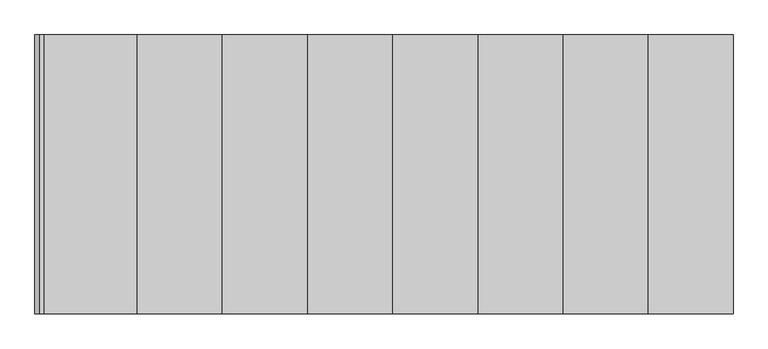
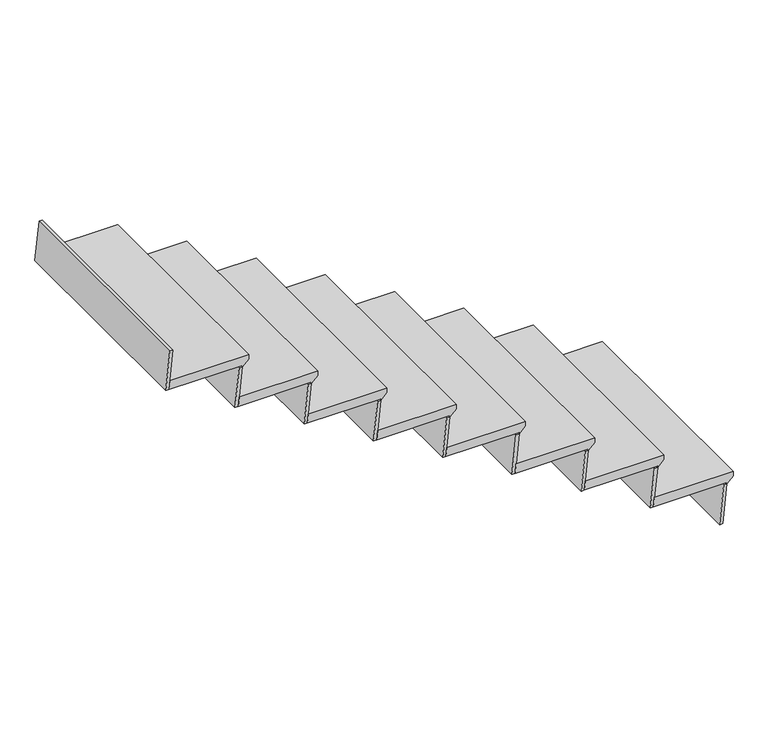
"""IFC4 building model written with IfcOpenShell, lengths in millimetres: stair flight geometry."""

import ifcopenshell
import ifcopenshell.guid

model = None  # the IFC model being written
_history = None  # IfcOwnerHistory: only IFC2X3 demands one
_inside = {}  # id of a spatial element -> (the spatial element, [elements in it])
_under = {}  # id of a project, library or spatial element -> (it, [spatial elements below it])
_declared = {}  # id of a project -> (the project, [libraries it declares])
_typed = {}  # id of a type object -> (the type object, [elements of that type])
_made_of = {}  # id of a material, layer set ... -> (it, [elements and type objects made of it])


def new_model(schema):
    """Start an empty IFC model of exactly this schema.

    Asked for "IFC4X3", IfcOpenShell would pick the latest addendum, in which some entities
    have other attributes; the version numbers below select the first issue.
    IFC2X3 requires an IfcOwnerHistory on every rooted entity: one is made here for all.
    """
    global model, _history
    if schema == "IFC4X3":
        model = ifcopenshell.file(schema_version=(4, 3, 0, 0))
    else:
        model = ifcopenshell.file(schema=schema)
    _inside.clear()
    _under.clear()
    _declared.clear()
    _typed.clear()
    _made_of.clear()
    _history = None
    if model.schema == "IFC2X3":
        org = make("IfcOrganization", Name="unknown")
        user = make(
            "IfcPersonAndOrganization",
            ThePerson=make("IfcPerson", FamilyName="unknown"),
            TheOrganization=org,
        )
        app = make(
            "IfcApplication",
            ApplicationDeveloper=org,
            Version="unknown",
            ApplicationFullName="unknown",
            ApplicationIdentifier="unknown",
        )
        _history = make(
            "IfcOwnerHistory",
            OwningUser=user,
            OwningApplication=app,
            ChangeAction="ADDED",
            CreationDate=0,
        )
    return model


def make(cls, **values):
    """One entity of the class cls with the attributes given. An attribute that is None is left unset."""
    return model.create_entity(
        cls, **{name: value for name, value in values.items() if value is not None}
    )


def rooted(cls, **values):
    """An entity with a GlobalId (a new one), such as an element, a storey or a relation."""
    return make(cls, GlobalId=ifcopenshell.guid.new(), OwnerHistory=_history, **values)


def si_unit(unit_type, name, prefix=None):
    """IfcSIUnit, for example si_unit("LENGTHUNIT", "METRE", prefix="MILLI")."""
    return make("IfcSIUnit", UnitType=unit_type, Prefix=prefix, Name=name)


def assignment(units):
    """IfcUnitAssignment: the units of a project."""
    return None if units is None else make("IfcUnitAssignment", Units=units)


def point(xyz):
    """IfcCartesianPoint."""
    return None if xyz is None else make("IfcCartesianPoint", Coordinates=xyz)


def direction(xyz):
    """IfcDirection."""
    return None if xyz is None else make("IfcDirection", DirectionRatios=xyz)


def frame(location, z_axis=None, x_axis=None):
    """IfcAxis2Placement3D, a coordinate frame: its origin and axes. An axis left out is left unset."""
    return make(
        "IfcAxis2Placement3D",
        Location=point(location),
        Axis=direction(z_axis),
        RefDirection=direction(x_axis),
    )


def origin():
    """The frame at (0, 0, 0) with its axes left unset."""
    return frame((0.0, 0.0, 0.0))


def place(relative_to, where):
    """IfcLocalPlacement: puts the frame where relative to a parent placement (None: the world)."""
    return make(
        "IfcLocalPlacement", PlacementRelTo=relative_to, RelativePlacement=where
    )


def context(
    kind, dimensions, precision=None, world=None, true_north=None, identifier=None
):
    """IfcGeometricRepresentationContext, for example the 3D "Model" context."""
    return make(
        "IfcGeometricRepresentationContext",
        ContextIdentifier=identifier,
        ContextType=kind,
        CoordinateSpaceDimension=dimensions,
        Precision=precision,
        WorldCoordinateSystem=world,
        TrueNorth=true_north,
    )


def project(units=None, contexts=None):
    """IfcProject with its units and contexts."""
    return rooted(
        "IfcProject",
        Name="project",
        RepresentationContexts=contexts,
        UnitsInContext=assignment(units),
    )


def spatial(cls, under=None, at=None, **own):
    """A site, building, storey or space (cls), placed at a placement, below another one or the project."""
    s = rooted(cls, ObjectPlacement=at, **own)
    if under is not None:
        _under.setdefault(under.id(), (under, []))[1].append(s)
    return s


def polyline(points):
    """IfcPolyline through the points."""
    return make("IfcPolyline", Points=[point(p) for p in points])


def outline(outer, holes=None, kind="AREA"):
    """IfcArbitraryClosedProfileDef: a profile drawn as a closed curve; with holes, ...WithVoids."""
    if holes is None:
        return make("IfcArbitraryClosedProfileDef", ProfileType=kind, OuterCurve=outer)
    return make(
        "IfcArbitraryProfileDefWithVoids",
        ProfileType=kind,
        OuterCurve=outer,
        InnerCurves=holes,
    )


def extrude(swept, where, along, depth):
    """IfcExtrudedAreaSolid: the profile swept, set in the frame where, extruded along a direction by depth."""
    return make(
        "IfcExtrudedAreaSolid",
        SweptArea=swept,
        Position=where,
        ExtrudedDirection=direction(along),
        Depth=depth,
    )


def shape(context_of_items, identifier, shape_type, items):
    """IfcShapeRepresentation: the items that make up one representation, for example the "Body"."""
    return make(
        "IfcShapeRepresentation",
        ContextOfItems=context_of_items,
        RepresentationIdentifier=identifier,
        RepresentationType=shape_type,
        Items=items,
    )


def source(mapping_origin, context_of_items, identifier, shape_type, items):
    """IfcRepresentationMap: a shape defined once, which mapped items show again and again."""
    return make(
        "IfcRepresentationMap",
        MappingOrigin=mapping_origin,
        MappedRepresentation=shape(context_of_items, identifier, shape_type, items),
    )


def transform(
    local_origin,
    x_axis=None,
    y_axis=None,
    z_axis=None,
    scale=None,
    scale2=None,
    scale3=None,
    uniform=True,
):
    """IfcCartesianTransformationOperator3D, or its non-uniform kind. x_axis, y_axis, z_axis: its Axis1, 2, 3."""
    if uniform:
        return make(
            "IfcCartesianTransformationOperator3D",
            Axis1=direction(x_axis),
            Axis2=direction(y_axis),
            LocalOrigin=point(local_origin),
            Scale=scale,
            Axis3=direction(z_axis),
        )
    return make(
        "IfcCartesianTransformationOperator3DnonUniform",
        Axis1=direction(x_axis),
        Axis2=direction(y_axis),
        LocalOrigin=point(local_origin),
        Scale=scale,
        Axis3=direction(z_axis),
        Scale2=scale2,
        Scale3=scale3,
    )


def mapped(mapping_source, mapping_target):
    """IfcMappedItem: shows the shape of a source again, moved by a transform."""
    return make(
        "IfcMappedItem", MappingSource=mapping_source, MappingTarget=mapping_target
    )


def made_of(thing, what):
    """Note that an element or type object is made of a material, layer set ...; save() writes the relation."""
    if what is not None:
        _made_of.setdefault(what.id(), (what, []))[1].append(thing)
    return thing


def element(
    cls,
    number,
    at=None,
    inside=None,
    cuts=None,
    type_object=None,
    material=None,
    context=None,
    identifier="Body",
    shape_type=None,
    held_by="IfcProductDefinitionShape",
    body=None,
    shapes=None,
    **own,
):
    """One element of the class cls, such as IfcWall. Its Tag is "e" and its number.

    at: its placement. inside: the storey or other place that contains it. cuts: it is an
    opening in that element (IfcRelVoidsElement). A single representation is given by context,
    identifier, shape_type and body (its items); several are given by shapes. held_by: the class
    of the entity that holds the representations. save() writes the other relations.
    """
    e = rooted(cls, Tag="e%d" % number, ObjectPlacement=at, **own)
    if body is not None:
        shapes = [shape(context, identifier, shape_type, body)]
    if shapes is not None:
        e.Representation = make(held_by, Representations=shapes)
    if inside is not None:
        _inside.setdefault(inside.id(), (inside, []))[1].append(e)
    if cuts is not None:
        rooted(
            "IfcRelVoidsElement", RelatingBuildingElement=cuts, RelatedOpeningElement=e
        )
    if type_object is not None:
        _typed.setdefault(type_object.id(), (type_object, []))[1].append(e)
    return made_of(e, material)


def aggregate(whole, parts):
    """IfcRelAggregates: a whole, such as a stair, and the parts it consists of."""
    return rooted("IfcRelAggregates", RelatingObject=whole, RelatedObjects=parts)


def save(model, path):
    """Write the relations noted so far, then the file.

    IfcRelAggregates (storeys below a building ...), IfcRelContainedInSpatialStructure (elements
    in a storey), IfcRelDefinesByType, IfcRelAssociatesMaterial and IfcRelDeclares: one each for
    every whole, place, type object, material and project.
    """
    for whole, parts in _under.values():
        aggregate(whole, parts)
    for where, things in _inside.values():
        rooted(
            "IfcRelContainedInSpatialStructure",
            RelatedElements=things,
            RelatingStructure=where,
        )
    for kind, things in _typed.values():
        rooted("IfcRelDefinesByType", RelatedObjects=things, RelatingType=kind)
    for what, things in _made_of.values():
        rooted("IfcRelAssociatesMaterial", RelatedObjects=things, RelatingMaterial=what)
    for by, libraries in _declared.values():
        rooted("IfcRelDeclares", RelatingContext=by, RelatedDefinitions=libraries)
    model.write(path)


def stair_flight_a5da1dd9(model_context):
    return source(origin(), model_context, "Body", "SweptSolid", [
        extrude(outline(polyline([(1693.3333333, -15521.4481446), (1693.3333333, -15838.9481446), (1655.2333333, -15842.8227209), (1655.2333333, -15546.8481446), (1648.8833333, -15546.8481446), (1674.2833333, -15521.4481446), (1693.3333333, -15521.4481446)])), frame((0.0, 17274.7635042, 0.0), z_axis=(0.0, 1.0, 0.0), x_axis=(0.0, 0.0, 1.0)), (0.0, 0.0, 1.0), 914.4),
        extrude(outline(polyline([(1648.8833333, -15546.8481446), (1648.8833333, -15559.6136465), (1485.9, -15576.1882228), (1485.9, -15563.4227209), (1648.8833333, -15546.8481446)])), frame((0.0, 17274.7635042, 0.0), z_axis=(0.0, 1.0, 0.0), x_axis=(0.0, 0.0, 1.0)), (0.0, 0.0, 1.0), 914.4),
        extrude(outline(polyline([(1818.2166667, -15826.2481446), (1818.2166667, -15839.0136465), (1655.2333333, -15855.5882228), (1655.2333333, -15842.8227209), (1818.2166667, -15826.2481446)])), frame((0.0, 17274.7635042, 0.0), z_axis=(0.0, 1.0, 0.0), x_axis=(0.0, 0.0, 1.0)), (0.0, 0.0, 1.0), 914.4),
        extrude(outline(polyline([(1862.6666667, -15800.8481446), (1862.6666667, -16118.3481446), (1824.5666667, -16122.2227209), (1824.5666667, -15826.2481446), (1818.2166667, -15826.2481446), (1843.6166667, -15800.8481446), (1862.6666667, -15800.8481446)])), frame((0.0, 17274.7635042, 0.0), z_axis=(0.0, 1.0, 0.0), x_axis=(0.0, 0.0, 1.0)), (0.0, 0.0, 1.0), 914.4),
        extrude(outline(polyline([(1987.55, -16105.6481446), (1987.55, -16118.4136465), (1824.5666667, -16134.9882228), (1824.5666667, -16122.2227209), (1987.55, -16105.6481446)])), frame((0.0, 17274.7635042, 0.0), z_axis=(0.0, 1.0, 0.0), x_axis=(0.0, 0.0, 1.0)), (0.0, 0.0, 1.0), 914.4),
        extrude(outline(polyline([(2032.0, -16080.2481446), (2032.0, -16397.7481446), (1993.9, -16401.6227209), (1993.9, -16105.6481446), (1987.55, -16105.6481446), (2012.95, -16080.2481446), (2032.0, -16080.2481446)])), frame((0.0, 17274.7635042, 0.0), z_axis=(0.0, 1.0, 0.0), x_axis=(0.0, 0.0, 1.0)), (0.0, 0.0, 1.0), 914.4),
        extrude(outline(polyline([(2156.8833333, -16385.0481446), (2156.8833333, -16397.8136465), (1993.9, -16414.3882228), (1993.9, -16401.6227209), (2156.8833333, -16385.0481446)])), frame((0.0, 17274.7635042, 0.0), z_axis=(0.0, 1.0, 0.0), x_axis=(0.0, 0.0, 1.0)), (0.0, 0.0, 1.0), 914.4),
        extrude(outline(polyline([(2201.3333333, -16359.6481446), (2201.3333333, -16677.1481446), (2163.2333333, -16681.0227209), (2163.2333333, -16385.0481446), (2156.8833333, -16385.0481446), (2182.2833333, -16359.6481446), (2201.3333333, -16359.6481446)])), frame((0.0, 17274.7635042, 0.0), z_axis=(0.0, 1.0, 0.0), x_axis=(0.0, 0.0, 1.0)), (0.0, 0.0, 1.0), 914.4),
        extrude(outline(polyline([(2326.2166667, -16664.4481446), (2326.2166667, -16677.2136465), (2163.2333333, -16693.7882228), (2163.2333333, -16681.0227209), (2326.2166667, -16664.4481446)])), frame((0.0, 17274.7635042, 0.0), z_axis=(0.0, 1.0, 0.0), x_axis=(0.0, 0.0, 1.0)), (0.0, 0.0, 1.0), 914.4),
        extrude(outline(polyline([(2370.6666667, -16639.0481446), (2370.6666667, -16956.5481446), (2332.5666667, -16960.4227209), (2332.5666667, -16664.4481446), (2326.2166667, -16664.4481446), (2351.6166667, -16639.0481446), (2370.6666667, -16639.0481446)])), frame((0.0, 17274.7635042, 0.0), z_axis=(0.0, 1.0, 0.0), x_axis=(0.0, 0.0, 1.0)), (0.0, 0.0, 1.0), 914.4),
        extrude(outline(polyline([(2495.55, -16943.8481446), (2495.55, -16956.6136465), (2332.5666667, -16973.1882228), (2332.5666667, -16960.4227209), (2495.55, -16943.8481446)])), frame((0.0, 17274.7635042, 0.0), z_axis=(0.0, 1.0, 0.0), x_axis=(0.0, 0.0, 1.0)), (0.0, 0.0, 1.0), 914.4),
        extrude(outline(polyline([(2540.0, -16918.4481446), (2540.0, -17235.9481446), (2501.9, -17239.8227209), (2501.9, -16943.8481446), (2495.55, -16943.8481446), (2520.95, -16918.4481446), (2540.0, -16918.4481446)])), frame((0.0, 17274.7635042, 0.0), z_axis=(0.0, 1.0, 0.0), x_axis=(0.0, 0.0, 1.0)), (0.0, 0.0, 1.0), 914.4),
        extrude(outline(polyline([(2664.8833333, -17223.2481446), (2664.8833333, -17236.0136465), (2501.9, -17252.5882228), (2501.9, -17239.8227209), (2664.8833333, -17223.2481446)])), frame((0.0, 17274.7635042, 0.0), z_axis=(0.0, 1.0, 0.0), x_axis=(0.0, 0.0, 1.0)), (0.0, 0.0, 1.0), 914.4),
        extrude(outline(polyline([(2709.3333333, -17197.8481446), (2709.3333333, -17515.3481446), (2671.2333333, -17519.2227209), (2671.2333333, -17223.2481446), (2664.8833333, -17223.2481446), (2690.2833333, -17197.8481446), (2709.3333333, -17197.8481446)])), frame((0.0, 17274.7635042, 0.0), z_axis=(0.0, 1.0, 0.0), x_axis=(0.0, 0.0, 1.0)), (0.0, 0.0, 1.0), 914.4),
        extrude(outline(polyline([(2834.2166667, -17502.6481446), (2834.2166667, -17515.4136465), (2671.2333333, -17531.9882228), (2671.2333333, -17519.2227209), (2834.2166667, -17502.6481446)])), frame((0.0, 17274.7635042, 0.0), z_axis=(0.0, 1.0, 0.0), x_axis=(0.0, 0.0, 1.0)), (0.0, 0.0, 1.0), 914.4),
        extrude(outline(polyline([(3003.55, -17782.0481446), (3003.55, -17794.8136465), (2840.5666667, -17811.3882228), (2840.5666667, -17798.6227209), (3003.55, -17782.0481446)])), frame((0.0, 17274.7635042, 0.0), z_axis=(0.0, 1.0, 0.0), x_axis=(0.0, 0.0, 1.0)), (0.0, 0.0, 1.0), 914.4),
        extrude(outline(polyline([(2878.6666667, -17477.2481446), (2878.6666667, -17794.7481446), (2840.5666667, -17798.6227209), (2840.5666667, -17502.6481446), (2834.2166667, -17502.6481446), (2859.6166667, -17477.2481446), (2878.6666667, -17477.2481446)])), frame((0.0, 17274.7635042, 0.0), z_axis=(0.0, 1.0, 0.0), x_axis=(0.0, 0.0, 1.0)), (0.0, 0.0, 1.0), 914.4),
    ])


if __name__ == "__main__":
    model = new_model("IFC4")
    model_context = context("Model", 3, world=origin())
    ifc_project = project(units=[si_unit("LENGTHUNIT", "METRE", prefix="MILLI")], contexts=[model_context])
    site = spatial("IfcSite", under=ifc_project)
    building = spatial("IfcBuilding", under=site)
    placement = place(None, origin())
    stair_flight_shape = stair_flight_a5da1dd9(model_context)
    element("IfcStairFlight", 1, at=placement, inside=building, context=model_context, shape_type="MappedRepresentation", body=[
        mapped(stair_flight_shape, transform((0.0, 0.0, 0.0), x_axis=(1.0, 0.0, 0.0), y_axis=(0.0, 1.0, 0.0), z_axis=(0.0, 0.0, 1.0))),
    ])
    save(model, "model.ifc")

# Revit data of these elements
# Element 1 (IfcStairFlight)
#   Materials on its faces: "Concrete - Cast-in-Place Concrete", "Metal - Paint Finish - Dark Gray, Matte"
# Materials
#   "Concrete - Cast-in-Place Concrete": class "Unassigned", colour RGB 192 192 192, transparency 0
#   "Metal - Paint Finish - Dark Gray, Matte": class "Unassigned", colour RGB 98 98 98, transparency 0
